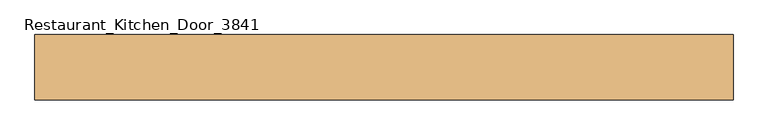
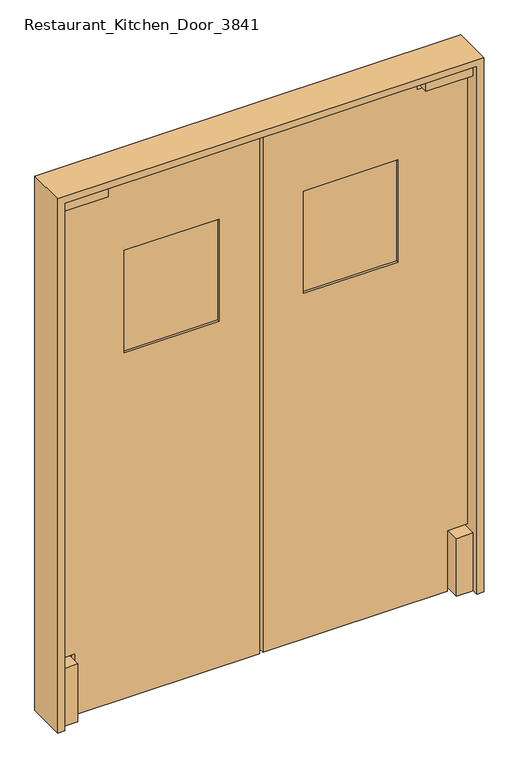
"""IFC4 building model written with IfcOpenShell, lengths in millimetres: door geometry, Restaurant_Kitchen_Door_3841."""

from ifc_helpers import new_model, si_unit, frame, origin, origin_with_axes, place, context, project, spatial, polyline, outline, extrude, source, transform, mapped, element, save


def restaurant_kitchen_door_3841_4c7ee789(model_context):
    return source(origin(), model_context, "Body", "SweptSolid", [
        extrude(outline(polyline([(0.0, -800.0), (0.0, -774.6), (2094.6, -774.6), (2094.6, 774.6), (0.0, 774.6), (0.0, 800.0), (2120.0, 800.0), (2120.0, -800.0), (0.0, -800.0)])), frame((0.0, -75.0, 0.0), z_axis=(0.0, 1.0, 0.0), x_axis=(0.0, 0.0, 1.0)), (0.0, 0.0, 1.0), 150.0),
        extrude(outline(polyline([(-596.8, -50.8), (-774.6, -50.8), (-774.6, 50.8), (-596.8, 50.8), (-596.8, -50.8)])), frame((0.0, 0.0, 2043.8), z_axis=(0.0, 0.0, 1.0), x_axis=(1.0, 0.0, 0.0)), (0.0, 0.0, 1.0), 50.8),
        extrude(outline(polyline([(774.6, -50.8), (596.8, -50.8), (596.8, 50.8), (774.6, 50.8), (774.6, -50.8)])), frame((0.0, 0.0, 2043.8), z_axis=(0.0, 0.0, 1.0), x_axis=(1.0, 0.0, 0.0)), (0.0, 0.0, 1.0), 50.8),
        extrude(outline(polyline([(774.6, -50.8), (711.1, -50.8), (711.1, 50.8), (774.6, 50.8), (774.6, -50.8)])), origin_with_axes(), (0.0, 0.0, 1.0), 228.6),
        extrude(outline(polyline([(-711.1, -50.8), (-774.6, -50.8), (-774.6, 50.8), (-711.1, 50.8), (-711.1, -50.8)])), origin_with_axes(), (0.0, 0.0, 1.0), 228.6),
        extrude(outline(polyline([(-158.75, -3.175), (-514.35, -3.175), (-514.35, 3.175), (-158.75, 3.175), (-158.75, -3.175)])), frame((0.0, 0.0, 1371.6), z_axis=(0.0, 0.0, 1.0), x_axis=(1.0, 0.0, 0.0)), (0.0, 0.0, 1.0), 406.4),
        extrude(outline(polyline([(2031.1, -774.6), (241.3, -774.6), (241.3, -698.4), (0.0, -698.4), (0.0, -6.35), (2094.6, -6.35), (2094.6, -584.1), (2031.1, -584.1), (2031.1, -774.6)]), holes=[polyline([(1778.0, -514.35), (1778.0, -158.75), (1371.6, -158.75), (1371.6, -514.35), (1778.0, -514.35)])]), frame((0.0, -12.7, 0.0), z_axis=(0.0, 1.0, 0.0), x_axis=(0.0, 0.0, 1.0)), (0.0, 0.0, 1.0), 25.4),
        extrude(outline(polyline([(514.35, -3.175), (158.75, -3.175), (158.75, 3.175), (514.35, 3.175), (514.35, -3.175)])), frame((0.0, 0.0, 1371.6), z_axis=(0.0, 0.0, 1.0), x_axis=(1.0, 0.0, 0.0)), (0.0, 0.0, 1.0), 406.4),
        extrude(outline(polyline([(2031.1, 774.6), (2031.1, 584.1), (2094.6, 584.1), (2094.6, 6.35), (0.0, 6.35), (0.0, 698.4), (241.3, 698.4), (241.3, 774.6), (2031.1, 774.6)]), holes=[polyline([(1371.6, 158.75), (1778.0, 158.75), (1778.0, 514.35), (1371.6, 514.35), (1371.6, 158.75)])]), frame((0.0, -12.7, 0.0), z_axis=(0.0, 1.0, 0.0), x_axis=(0.0, 0.0, 1.0)), (0.0, 0.0, 1.0), 25.4),
    ])


if __name__ == "__main__":
    model = new_model("IFC4")
    model_context = context("Model", 3, world=origin())
    ifc_project = project(units=[si_unit("LENGTHUNIT", "METRE", prefix="MILLI")], contexts=[model_context])
    site = spatial("IfcSite", under=ifc_project)
    building = spatial("IfcBuilding", under=site)
    placement = place(None, origin())
    restaurant_kitchen_door_3841_shape = restaurant_kitchen_door_3841_4c7ee789(model_context)
    element("IfcDoor", 1, ObjectType="Restaurant_Kitchen_Door_3841 : 5'-4\"W. x 7'-2\"H.", at=placement, inside=building, context=model_context, shape_type="MappedRepresentation", body=[
        mapped(restaurant_kitchen_door_3841_shape, transform((0.0, 0.0, 0.0), x_axis=(1.0, 0.0, 0.0), y_axis=(0.0, 1.0, 0.0), z_axis=(0.0, 0.0, 1.0))),
    ])
    save(model, "model.ifc")

# Revit data of these elements
# Type "Restaurant_Kitchen_Door_3841 : 5'-4\"W. x 7'-2\"H."
#   Type Mark = "C26"
#   Analytic Construction = "<Nenhum>"
#   Rough Width = 1600 mm
#   Rough Height = 2120 mm
#   Height = 2094.6 mm
#   Width = 774.6 mm
#   Define Thermal Properties by = 1
#   Glass = Glazing - Interior
#   Frame = Door - Kitchen - Frame
#   Door Panel = Door - Kitchen - Panel
#   Function = (empty or 0)
#   Wall Closure = (empty or 0)
# Element 1 (IfcDoor, "Restaurant_Kitchen_Door_3841 : 5'-4\"W. x 7'-2\"H.")
#   Materials on its faces: "Door - Kitchen - Frame", "Door - Kitchen - Panel", "Glazing - Interior"
# Materials
#   "Glazing - Interior": class "Não atribuído", colour RGB 0 0 255, transparency 0.75
#   "Door - Kitchen - Frame": class "Não atribuído", colour RGB 247 247 247, transparency 0
#   "Door - Kitchen - Panel": class "Não atribuído", colour RGB 50 50 50, transparency 0, Comments = "A aparência de renderização não foi atualizada "
